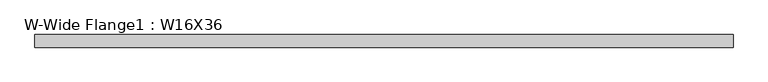
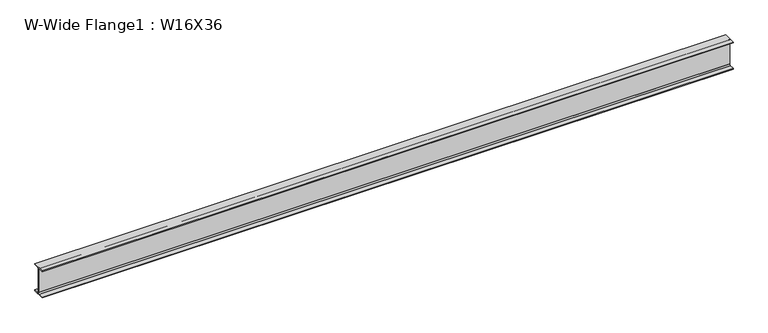
"""IFC4 building model written with IfcOpenShell, lengths in millimetres: beam geometry, W-Wide Flange1 : W16X36."""

import ifcopenshell
import ifcopenshell.guid

model = None  # the IFC model being written
_history = None  # IfcOwnerHistory: only IFC2X3 demands one
_inside = {}  # id of a spatial element -> (the spatial element, [elements in it])
_under = {}  # id of a project, library or spatial element -> (it, [spatial elements below it])
_declared = {}  # id of a project -> (the project, [libraries it declares])
_typed = {}  # id of a type object -> (the type object, [elements of that type])
_made_of = {}  # id of a material, layer set ... -> (it, [elements and type objects made of it])


def new_model(schema):
    """Start an empty IFC model of exactly this schema.

    Asked for "IFC4X3", IfcOpenShell would pick the latest addendum, in which some entities
    have other attributes; the version numbers below select the first issue.
    IFC2X3 requires an IfcOwnerHistory on every rooted entity: one is made here for all.
    """
    global model, _history
    if schema == "IFC4X3":
        model = ifcopenshell.file(schema_version=(4, 3, 0, 0))
    else:
        model = ifcopenshell.file(schema=schema)
    _inside.clear()
    _under.clear()
    _declared.clear()
    _typed.clear()
    _made_of.clear()
    _history = None
    if model.schema == "IFC2X3":
        org = make("IfcOrganization", Name="unknown")
        user = make(
            "IfcPersonAndOrganization",
            ThePerson=make("IfcPerson", FamilyName="unknown"),
            TheOrganization=org,
        )
        app = make(
            "IfcApplication",
            ApplicationDeveloper=org,
            Version="unknown",
            ApplicationFullName="unknown",
            ApplicationIdentifier="unknown",
        )
        _history = make(
            "IfcOwnerHistory",
            OwningUser=user,
            OwningApplication=app,
            ChangeAction="ADDED",
            CreationDate=0,
        )
    return model


def make(cls, **values):
    """One entity of the class cls with the attributes given. An attribute that is None is left unset."""
    return model.create_entity(
        cls, **{name: value for name, value in values.items() if value is not None}
    )


def rooted(cls, **values):
    """An entity with a GlobalId (a new one), such as an element, a storey or a relation."""
    return make(cls, GlobalId=ifcopenshell.guid.new(), OwnerHistory=_history, **values)


def si_unit(unit_type, name, prefix=None):
    """IfcSIUnit, for example si_unit("LENGTHUNIT", "METRE", prefix="MILLI")."""
    return make("IfcSIUnit", UnitType=unit_type, Prefix=prefix, Name=name)


def assignment(units):
    """IfcUnitAssignment: the units of a project."""
    return None if units is None else make("IfcUnitAssignment", Units=units)


def point(xyz):
    """IfcCartesianPoint."""
    return None if xyz is None else make("IfcCartesianPoint", Coordinates=xyz)


def direction(xyz):
    """IfcDirection."""
    return None if xyz is None else make("IfcDirection", DirectionRatios=xyz)


def frame(location, z_axis=None, x_axis=None):
    """IfcAxis2Placement3D, a coordinate frame: its origin and axes. An axis left out is left unset."""
    return make(
        "IfcAxis2Placement3D",
        Location=point(location),
        Axis=direction(z_axis),
        RefDirection=direction(x_axis),
    )


def frame_2d(location, x_axis=None):
    """IfcAxis2Placement2D, a coordinate frame in the plane: its origin and x axis."""
    return make(
        "IfcAxis2Placement2D", Location=point(location), RefDirection=direction(x_axis)
    )


def origin():
    """The frame at (0, 0, 0) with its axes left unset."""
    return frame((0.0, 0.0, 0.0))


def place(relative_to, where):
    """IfcLocalPlacement: puts the frame where relative to a parent placement (None: the world)."""
    return make(
        "IfcLocalPlacement", PlacementRelTo=relative_to, RelativePlacement=where
    )


def context(
    kind, dimensions, precision=None, world=None, true_north=None, identifier=None
):
    """IfcGeometricRepresentationContext, for example the 3D "Model" context."""
    return make(
        "IfcGeometricRepresentationContext",
        ContextIdentifier=identifier,
        ContextType=kind,
        CoordinateSpaceDimension=dimensions,
        Precision=precision,
        WorldCoordinateSystem=world,
        TrueNorth=true_north,
    )


def project(units=None, contexts=None):
    """IfcProject with its units and contexts."""
    return rooted(
        "IfcProject",
        Name="project",
        RepresentationContexts=contexts,
        UnitsInContext=assignment(units),
    )


def spatial(cls, under=None, at=None, **own):
    """A site, building, storey or space (cls), placed at a placement, below another one or the project."""
    s = rooted(cls, ObjectPlacement=at, **own)
    if under is not None:
        _under.setdefault(under.id(), (under, []))[1].append(s)
    return s


def polyline(points):
    """IfcPolyline through the points."""
    return make("IfcPolyline", Points=[point(p) for p in points])


def circle_curve(where, radius):
    """IfcCircle in the frame where."""
    return make("IfcCircle", Position=where, Radius=radius)


def trimmed(basis, trim1, trim2, sense, master):
    """IfcTrimmedCurve: the piece of a basis curve between two trims."""
    return make(
        "IfcTrimmedCurve",
        BasisCurve=basis,
        Trim1=trim1,
        Trim2=trim2,
        SenseAgreement=sense,
        MasterRepresentation=master,
    )


def segment(curve, same_sense, transition):
    """IfcCompositeCurveSegment."""
    return make(
        "IfcCompositeCurveSegment",
        Transition=transition,
        SameSense=same_sense,
        ParentCurve=curve,
    )


def composite_curve(segments, self_intersect=None):
    """IfcCompositeCurve: segments joined end to end."""
    return make("IfcCompositeCurve", Segments=segments, SelfIntersect=self_intersect)


def outline(outer, holes=None, kind="AREA"):
    """IfcArbitraryClosedProfileDef: a profile drawn as a closed curve; with holes, ...WithVoids."""
    if holes is None:
        return make("IfcArbitraryClosedProfileDef", ProfileType=kind, OuterCurve=outer)
    return make(
        "IfcArbitraryProfileDefWithVoids",
        ProfileType=kind,
        OuterCurve=outer,
        InnerCurves=holes,
    )


def extrude(swept, where, along, depth):
    """IfcExtrudedAreaSolid: the profile swept, set in the frame where, extruded along a direction by depth."""
    return make(
        "IfcExtrudedAreaSolid",
        SweptArea=swept,
        Position=where,
        ExtrudedDirection=direction(along),
        Depth=depth,
    )


def shape(context_of_items, identifier, shape_type, items):
    """IfcShapeRepresentation: the items that make up one representation, for example the "Body"."""
    return make(
        "IfcShapeRepresentation",
        ContextOfItems=context_of_items,
        RepresentationIdentifier=identifier,
        RepresentationType=shape_type,
        Items=items,
    )


def source(mapping_origin, context_of_items, identifier, shape_type, items):
    """IfcRepresentationMap: a shape defined once, which mapped items show again and again."""
    return make(
        "IfcRepresentationMap",
        MappingOrigin=mapping_origin,
        MappedRepresentation=shape(context_of_items, identifier, shape_type, items),
    )


def transform(
    local_origin,
    x_axis=None,
    y_axis=None,
    z_axis=None,
    scale=None,
    scale2=None,
    scale3=None,
    uniform=True,
):
    """IfcCartesianTransformationOperator3D, or its non-uniform kind. x_axis, y_axis, z_axis: its Axis1, 2, 3."""
    if uniform:
        return make(
            "IfcCartesianTransformationOperator3D",
            Axis1=direction(x_axis),
            Axis2=direction(y_axis),
            LocalOrigin=point(local_origin),
            Scale=scale,
            Axis3=direction(z_axis),
        )
    return make(
        "IfcCartesianTransformationOperator3DnonUniform",
        Axis1=direction(x_axis),
        Axis2=direction(y_axis),
        LocalOrigin=point(local_origin),
        Scale=scale,
        Axis3=direction(z_axis),
        Scale2=scale2,
        Scale3=scale3,
    )


def mapped(mapping_source, mapping_target):
    """IfcMappedItem: shows the shape of a source again, moved by a transform."""
    return make(
        "IfcMappedItem", MappingSource=mapping_source, MappingTarget=mapping_target
    )


def made_of(thing, what):
    """Note that an element or type object is made of a material, layer set ...; save() writes the relation."""
    if what is not None:
        _made_of.setdefault(what.id(), (what, []))[1].append(thing)
    return thing


def element(
    cls,
    number,
    at=None,
    inside=None,
    cuts=None,
    type_object=None,
    material=None,
    context=None,
    identifier="Body",
    shape_type=None,
    held_by="IfcProductDefinitionShape",
    body=None,
    shapes=None,
    **own,
):
    """One element of the class cls, such as IfcWall. Its Tag is "e" and its number.

    at: its placement. inside: the storey or other place that contains it. cuts: it is an
    opening in that element (IfcRelVoidsElement). A single representation is given by context,
    identifier, shape_type and body (its items); several are given by shapes. held_by: the class
    of the entity that holds the representations. save() writes the other relations.
    """
    e = rooted(cls, Tag="e%d" % number, ObjectPlacement=at, **own)
    if body is not None:
        shapes = [shape(context, identifier, shape_type, body)]
    if shapes is not None:
        e.Representation = make(held_by, Representations=shapes)
    if inside is not None:
        _inside.setdefault(inside.id(), (inside, []))[1].append(e)
    if cuts is not None:
        rooted(
            "IfcRelVoidsElement", RelatingBuildingElement=cuts, RelatedOpeningElement=e
        )
    if type_object is not None:
        _typed.setdefault(type_object.id(), (type_object, []))[1].append(e)
    return made_of(e, material)


def aggregate(whole, parts):
    """IfcRelAggregates: a whole, such as a stair, and the parts it consists of."""
    return rooted("IfcRelAggregates", RelatingObject=whole, RelatedObjects=parts)


def save(model, path):
    """Write the relations noted so far, then the file.

    IfcRelAggregates (storeys below a building ...), IfcRelContainedInSpatialStructure (elements
    in a storey), IfcRelDefinesByType, IfcRelAssociatesMaterial and IfcRelDeclares: one each for
    every whole, place, type object, material and project.
    """
    for whole, parts in _under.values():
        aggregate(whole, parts)
    for where, things in _inside.values():
        rooted(
            "IfcRelContainedInSpatialStructure",
            RelatedElements=things,
            RelatingStructure=where,
        )
    for kind, things in _typed.values():
        rooted("IfcRelDefinesByType", RelatedObjects=things, RelatingType=kind)
    for what, things in _made_of.values():
        rooted("IfcRelAssociatesMaterial", RelatedObjects=things, RelatingMaterial=what)
    for by, libraries in _declared.values():
        rooted("IfcRelDeclares", RelatingContext=by, RelatedDefinitions=libraries)
    model.write(path)


def w_wide_flange1_w16x36_389d0f9a(model_context):
    return source(origin(), model_context, "Body", "SweptSolid", [
        extrude(outline(composite_curve([segment(polyline([(88.773, -191.008), (88.773, -201.93), (-88.773, -201.93), (-88.773, -191.008), (-21.3995, -191.008)]), True, "CONTINUOUS"), segment(trimmed(circle_curve(frame_2d((-21.3995, -173.355)), 17.653), [point((-21.3995, -191.008))], [point((-3.7465, -173.355))], True, "CARTESIAN"), True, "CONTINUOUS"), segment(polyline([(-3.7465, -173.355), (-3.7465, 173.355)]), True, "CONTINUOUS"), segment(trimmed(circle_curve(frame_2d((-21.3995, 173.355)), 17.653), [point((-3.7465, 173.355))], [point((-21.3995, 191.008))], True, "CARTESIAN"), True, "CONTINUOUS"), segment(polyline([(-21.3995, 191.008), (-88.773, 191.008), (-88.773, 201.93), (88.773, 201.93), (88.773, 191.008), (21.3995, 191.008)]), True, "CONTINUOUS"), segment(trimmed(circle_curve(frame_2d((21.3995, 173.355)), 17.653), [point((21.3995, 191.008))], [point((3.7465, 173.355))], True, "CARTESIAN"), True, "CONTINUOUS"), segment(polyline([(3.7465, 173.355), (3.7465, -173.355)]), True, "CONTINUOUS"), segment(trimmed(circle_curve(frame_2d((21.3995, -173.355)), 17.653), [point((3.7465, -173.355))], [point((21.3995, -191.008))], True, "CARTESIAN"), True, "CONTINUOUS"), segment(polyline([(21.3995, -191.008), (88.773, -191.008)]), True, "CONTINUOUS")], self_intersect=False)), frame((-4901.0159349, 0.0, 0.0), z_axis=(1.0, 0.0, 0.0), x_axis=(0.0, 1.0, 0.0)), (0.0, 0.0, 1.0), 9802.0318698),
    ])


if __name__ == "__main__":
    model = new_model("IFC4")
    model_context = context("Model", 3, world=origin())
    ifc_project = project(units=[si_unit("LENGTHUNIT", "METRE", prefix="MILLI")], contexts=[model_context])
    site = spatial("IfcSite", under=ifc_project)
    building = spatial("IfcBuilding", under=site)
    placement = place(None, origin())
    w_wide_flange1_w16x36_shape = w_wide_flange1_w16x36_389d0f9a(model_context)
    element("IfcBeam", 1, ObjectType="W-Wide Flange1 : W16X36", at=placement, inside=building, context=model_context, shape_type="MappedRepresentation", body=[
        mapped(w_wide_flange1_w16x36_shape, transform((0.0, 0.0, 0.0), x_axis=(1.0, 0.0, 0.0), y_axis=(0.0, 1.0, 0.0), z_axis=(0.0, 0.0, 1.0))),
    ])
    save(model, "model.ifc")

# Revit data of these elements
# Type "W-Wide Flange1 : W16X36"
#   Assembly Code = "B10"
#   W = 36
#   Start Extension Calculation [instance default] = 10' - 0"
#   Start Extension [instance default] = -0' - 0 1/2"
#   End Extension Calculation [instance default] = 10' - 0"
#   End Extension [instance default] = -0' - 0 1/2"
#   Length [instance default] = 5' - 0"
#   bf = 0' - 6.99"
#   d = 1' - 3.9"
#   k = 0' - 1 1/8"
#   k2 = 0' - 0.695"
#   tf = 0' - 0.43"
#   tw = 0' - 0.295"
#   A = 0.0736111 SF
#   Structural Material [instance default] = Metal - Steel - ASTM A992
# Element 1 (IfcBeam, "W-Wide Flange1 : W16X36")
#   Materials on its faces: "Metal - Steel - ASTM A992"
# Materials
#   "Metal - Steel - ASTM A992": class "Metal", colour RGB 199 199 199, transparency 0
